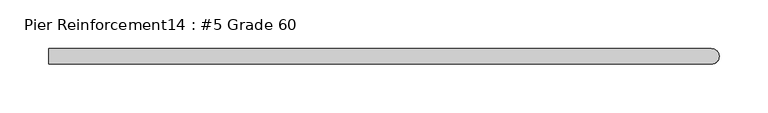
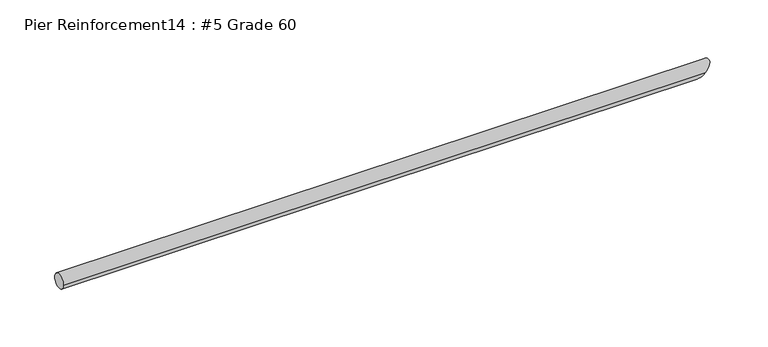
"""IFC4 building model written with IfcOpenShell, lengths in millimetres: proxy geometry, Pier Reinforcement14 : #5 Grade 60."""

from ifc_helpers import new_model, si_unit, frame, origin, place, context, project, spatial, circle_curve, ellipse_curve, source, transform, mapped, element, save
from ifc_brep_helpers import plane_surface, cylinder_surface, advanced_brep


def pier_reinforcement14_5_grade_60_09892ae6(model_context):
    return source(origin(), model_context, "Body", "AdvancedBrep", [
        advanced_brep(
        [(589548.1922365, -534037.9288841, -55.5625), (589548.1922365, -534053.8038841, -55.5625), (590226.0547365, -534053.8038841, -55.5625), (590233.9922365, -534045.8663841, -47.625), (590226.0547365, -534037.9288841, -55.5625), (590218.1172365, -534045.8663841, -63.5)],
        [
            (0, 1, circle_curve(frame((589548.1922365, -534045.8663841, -55.5625), z_axis=(-1.0, 0.0, 0.0), x_axis=(0.0, -1.0, 0.0)), 7.9375)),
            (1, 0, circle_curve(frame((589548.1922365, -534045.8663841, -55.5625), z_axis=(-1.0, 0.0, 0.0), x_axis=(0.0, -1.0, 0.0)), 7.9375)),
            (1, 2),
            (2, 3, ellipse_curve(frame((590226.0547365, -534045.8663841, -55.5625), z_axis=(-0.7071067811865462, 0.0, 0.7071067811865489), x_axis=(0.7071067811865487, 0.0, 0.7071067811865462)), 11.2253202, 7.9375)),
            (3, 4, ellipse_curve(frame((590226.0547365, -534045.8663841, -55.5625), z_axis=(-0.7071067811865462, 0.0, 0.7071067811865489), x_axis=(0.7071067811865487, 0.0, 0.7071067811865462)), 11.2253202, 7.9375)),
            (4, 0),
            (4, 5, ellipse_curve(frame((590226.0547365, -534045.8663841, -55.5625), z_axis=(-0.7071067811865462, 0.0, 0.7071067811865489), x_axis=(0.7071067811865487, 0.0, 0.7071067811865462)), 11.2253202, 7.9375)),
            (5, 2, ellipse_curve(frame((590226.0547365, -534045.8663841, -55.5625), z_axis=(-0.7071067811865462, 0.0, 0.7071067811865489), x_axis=(0.7071067811865487, 0.0, 0.7071067811865462)), 11.2253202, 7.9375)),
        ],
        [
            plane_surface(frame((589548.1922365, -534053.8038841, -55.5625), z_axis=(-1.0, 0.0, 0.0), x_axis=(0.0, 0.0, 1.0))),
            cylinder_surface(frame((589548.1922365, -534045.8663841, -55.5625), z_axis=(1.0, 0.0, 0.0), x_axis=(0.0, -1.0, 0.0)), 7.9375),
            plane_surface(frame((590218.1172365, -534020.4663841, -63.5), z_axis=(0.7071067811865462, 0.0, -0.7071067811865489), x_axis=(0.0, -1.0, 0.0))),
        ],
        [
            (0, [[1, 2]]),
            (1, [[-2, 3, 4, 5, 6]]),
            (1, [[-1, -6, 7, 8, -3]]),
            (2, [[-5, -4, -8, -7]]),
        ],
    ),
    ])


if __name__ == "__main__":
    model = new_model("IFC4")
    model_context = context("Model", 3, world=origin())
    ifc_project = project(units=[si_unit("LENGTHUNIT", "METRE", prefix="MILLI")], contexts=[model_context])
    site = spatial("IfcSite", under=ifc_project)
    building = spatial("IfcBuilding", under=site)
    placement = place(None, origin())
    pier_reinforcement14_5_grade_60_shape = pier_reinforcement14_5_grade_60_09892ae6(model_context)
    element("IfcBuildingElementProxy", 1, Name="Pier Reinforcement14 : #5 Grade 60", ObjectType="Pier Reinforcement14 : #5 Grade 60", at=placement, inside=building, context=model_context, shape_type="MappedRepresentation", body=[
        mapped(pier_reinforcement14_5_grade_60_shape, transform((0.0, 0.0, 0.0), x_axis=(1.0, 0.0, 0.0), y_axis=(0.0, 1.0, 0.0), z_axis=(0.0, 0.0, 1.0))),
    ])
    save(model, "model.ifc")

# Revit data of these elements
# Element 1 (IfcBuildingElementProxy, "Pier Reinforcement14 : #5 Grade 60")
#   Materials on its faces: "#5 GR. 60 BEND 24\"x24\""
# Materials
#   "#5 GR. 60 BEND 24\"x24\"": class "Generic", colour RGB 84 83 81, transparency 0, Cost = 0
